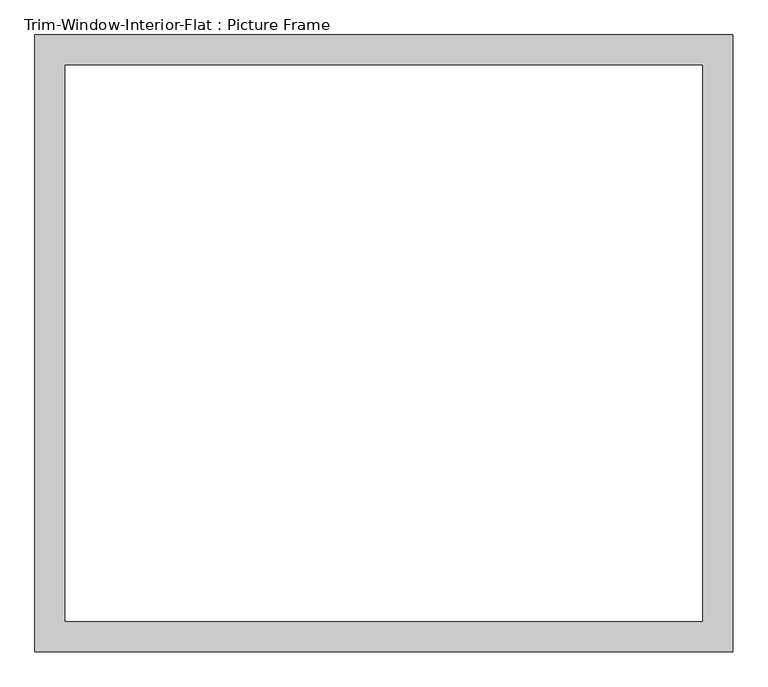
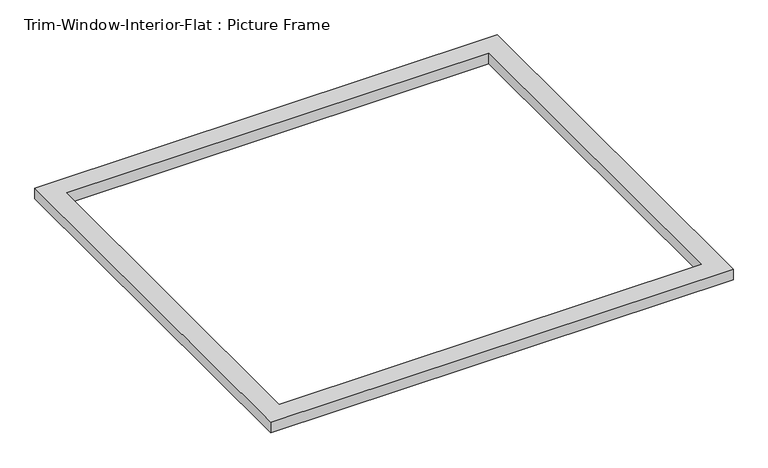
"""IFC4 building model written with IfcOpenShell, lengths in millimetres: proxy geometry, Trim-Window-Interior-Flat : Picture Frame."""

import ifcopenshell
import ifcopenshell.guid

model = None  # the IFC model being written
_history = None  # IfcOwnerHistory: only IFC2X3 demands one
_inside = {}  # id of a spatial element -> (the spatial element, [elements in it])
_under = {}  # id of a project, library or spatial element -> (it, [spatial elements below it])
_declared = {}  # id of a project -> (the project, [libraries it declares])
_typed = {}  # id of a type object -> (the type object, [elements of that type])
_made_of = {}  # id of a material, layer set ... -> (it, [elements and type objects made of it])


def new_model(schema):
    """Start an empty IFC model of exactly this schema.

    Asked for "IFC4X3", IfcOpenShell would pick the latest addendum, in which some entities
    have other attributes; the version numbers below select the first issue.
    IFC2X3 requires an IfcOwnerHistory on every rooted entity: one is made here for all.
    """
    global model, _history
    if schema == "IFC4X3":
        model = ifcopenshell.file(schema_version=(4, 3, 0, 0))
    else:
        model = ifcopenshell.file(schema=schema)
    _inside.clear()
    _under.clear()
    _declared.clear()
    _typed.clear()
    _made_of.clear()
    _history = None
    if model.schema == "IFC2X3":
        org = make("IfcOrganization", Name="unknown")
        user = make(
            "IfcPersonAndOrganization",
            ThePerson=make("IfcPerson", FamilyName="unknown"),
            TheOrganization=org,
        )
        app = make(
            "IfcApplication",
            ApplicationDeveloper=org,
            Version="unknown",
            ApplicationFullName="unknown",
            ApplicationIdentifier="unknown",
        )
        _history = make(
            "IfcOwnerHistory",
            OwningUser=user,
            OwningApplication=app,
            ChangeAction="ADDED",
            CreationDate=0,
        )
    return model


def make(cls, **values):
    """One entity of the class cls with the attributes given. An attribute that is None is left unset."""
    return model.create_entity(
        cls, **{name: value for name, value in values.items() if value is not None}
    )


def rooted(cls, **values):
    """An entity with a GlobalId (a new one), such as an element, a storey or a relation."""
    return make(cls, GlobalId=ifcopenshell.guid.new(), OwnerHistory=_history, **values)


def si_unit(unit_type, name, prefix=None):
    """IfcSIUnit, for example si_unit("LENGTHUNIT", "METRE", prefix="MILLI")."""
    return make("IfcSIUnit", UnitType=unit_type, Prefix=prefix, Name=name)


def assignment(units):
    """IfcUnitAssignment: the units of a project."""
    return None if units is None else make("IfcUnitAssignment", Units=units)


def point(xyz):
    """IfcCartesianPoint."""
    return None if xyz is None else make("IfcCartesianPoint", Coordinates=xyz)


def direction(xyz):
    """IfcDirection."""
    return None if xyz is None else make("IfcDirection", DirectionRatios=xyz)


def frame(location, z_axis=None, x_axis=None):
    """IfcAxis2Placement3D, a coordinate frame: its origin and axes. An axis left out is left unset."""
    return make(
        "IfcAxis2Placement3D",
        Location=point(location),
        Axis=direction(z_axis),
        RefDirection=direction(x_axis),
    )


def origin():
    """The frame at (0, 0, 0) with its axes left unset."""
    return frame((0.0, 0.0, 0.0))


def origin_with_axes():
    """The frame at (0, 0, 0) with the z axis (0, 0, 1) and the x axis (1, 0, 0) written out."""
    return frame((0.0, 0.0, 0.0), z_axis=(0.0, 0.0, 1.0), x_axis=(1.0, 0.0, 0.0))


def place(relative_to, where):
    """IfcLocalPlacement: puts the frame where relative to a parent placement (None: the world)."""
    return make(
        "IfcLocalPlacement", PlacementRelTo=relative_to, RelativePlacement=where
    )


def context(
    kind, dimensions, precision=None, world=None, true_north=None, identifier=None
):
    """IfcGeometricRepresentationContext, for example the 3D "Model" context."""
    return make(
        "IfcGeometricRepresentationContext",
        ContextIdentifier=identifier,
        ContextType=kind,
        CoordinateSpaceDimension=dimensions,
        Precision=precision,
        WorldCoordinateSystem=world,
        TrueNorth=true_north,
    )


def project(units=None, contexts=None):
    """IfcProject with its units and contexts."""
    return rooted(
        "IfcProject",
        Name="project",
        RepresentationContexts=contexts,
        UnitsInContext=assignment(units),
    )


def spatial(cls, under=None, at=None, **own):
    """A site, building, storey or space (cls), placed at a placement, below another one or the project."""
    s = rooted(cls, ObjectPlacement=at, **own)
    if under is not None:
        _under.setdefault(under.id(), (under, []))[1].append(s)
    return s


def polyline(points):
    """IfcPolyline through the points."""
    return make("IfcPolyline", Points=[point(p) for p in points])


def outline(outer, holes=None, kind="AREA"):
    """IfcArbitraryClosedProfileDef: a profile drawn as a closed curve; with holes, ...WithVoids."""
    if holes is None:
        return make("IfcArbitraryClosedProfileDef", ProfileType=kind, OuterCurve=outer)
    return make(
        "IfcArbitraryProfileDefWithVoids",
        ProfileType=kind,
        OuterCurve=outer,
        InnerCurves=holes,
    )


def extrude(swept, where, along, depth):
    """IfcExtrudedAreaSolid: the profile swept, set in the frame where, extruded along a direction by depth."""
    return make(
        "IfcExtrudedAreaSolid",
        SweptArea=swept,
        Position=where,
        ExtrudedDirection=direction(along),
        Depth=depth,
    )


def shape(context_of_items, identifier, shape_type, items):
    """IfcShapeRepresentation: the items that make up one representation, for example the "Body"."""
    return make(
        "IfcShapeRepresentation",
        ContextOfItems=context_of_items,
        RepresentationIdentifier=identifier,
        RepresentationType=shape_type,
        Items=items,
    )


def source(mapping_origin, context_of_items, identifier, shape_type, items):
    """IfcRepresentationMap: a shape defined once, which mapped items show again and again."""
    return make(
        "IfcRepresentationMap",
        MappingOrigin=mapping_origin,
        MappedRepresentation=shape(context_of_items, identifier, shape_type, items),
    )


def transform(
    local_origin,
    x_axis=None,
    y_axis=None,
    z_axis=None,
    scale=None,
    scale2=None,
    scale3=None,
    uniform=True,
):
    """IfcCartesianTransformationOperator3D, or its non-uniform kind. x_axis, y_axis, z_axis: its Axis1, 2, 3."""
    if uniform:
        return make(
            "IfcCartesianTransformationOperator3D",
            Axis1=direction(x_axis),
            Axis2=direction(y_axis),
            LocalOrigin=point(local_origin),
            Scale=scale,
            Axis3=direction(z_axis),
        )
    return make(
        "IfcCartesianTransformationOperator3DnonUniform",
        Axis1=direction(x_axis),
        Axis2=direction(y_axis),
        LocalOrigin=point(local_origin),
        Scale=scale,
        Axis3=direction(z_axis),
        Scale2=scale2,
        Scale3=scale3,
    )


def mapped(mapping_source, mapping_target):
    """IfcMappedItem: shows the shape of a source again, moved by a transform."""
    return make(
        "IfcMappedItem", MappingSource=mapping_source, MappingTarget=mapping_target
    )


def made_of(thing, what):
    """Note that an element or type object is made of a material, layer set ...; save() writes the relation."""
    if what is not None:
        _made_of.setdefault(what.id(), (what, []))[1].append(thing)
    return thing


def element(
    cls,
    number,
    at=None,
    inside=None,
    cuts=None,
    type_object=None,
    material=None,
    context=None,
    identifier="Body",
    shape_type=None,
    held_by="IfcProductDefinitionShape",
    body=None,
    shapes=None,
    **own,
):
    """One element of the class cls, such as IfcWall. Its Tag is "e" and its number.

    at: its placement. inside: the storey or other place that contains it. cuts: it is an
    opening in that element (IfcRelVoidsElement). A single representation is given by context,
    identifier, shape_type and body (its items); several are given by shapes. held_by: the class
    of the entity that holds the representations. save() writes the other relations.
    """
    e = rooted(cls, Tag="e%d" % number, ObjectPlacement=at, **own)
    if body is not None:
        shapes = [shape(context, identifier, shape_type, body)]
    if shapes is not None:
        e.Representation = make(held_by, Representations=shapes)
    if inside is not None:
        _inside.setdefault(inside.id(), (inside, []))[1].append(e)
    if cuts is not None:
        rooted(
            "IfcRelVoidsElement", RelatingBuildingElement=cuts, RelatedOpeningElement=e
        )
    if type_object is not None:
        _typed.setdefault(type_object.id(), (type_object, []))[1].append(e)
    return made_of(e, material)


def aggregate(whole, parts):
    """IfcRelAggregates: a whole, such as a stair, and the parts it consists of."""
    return rooted("IfcRelAggregates", RelatingObject=whole, RelatedObjects=parts)


def save(model, path):
    """Write the relations noted so far, then the file.

    IfcRelAggregates (storeys below a building ...), IfcRelContainedInSpatialStructure (elements
    in a storey), IfcRelDefinesByType, IfcRelAssociatesMaterial and IfcRelDeclares: one each for
    every whole, place, type object, material and project.
    """
    for whole, parts in _under.values():
        aggregate(whole, parts)
    for where, things in _inside.values():
        rooted(
            "IfcRelContainedInSpatialStructure",
            RelatedElements=things,
            RelatingStructure=where,
        )
    for kind, things in _typed.values():
        rooted("IfcRelDefinesByType", RelatedObjects=things, RelatingType=kind)
    for what, things in _made_of.values():
        rooted("IfcRelAssociatesMaterial", RelatedObjects=things, RelatingMaterial=what)
    for by, libraries in _declared.values():
        rooted("IfcRelDeclares", RelatingContext=by, RelatedDefinitions=libraries)
    model.write(path)


def trim_window_interior_flat_picture_frame_1dce1945(model_context):
    return source(origin(), model_context, "Body", "SweptSolid", [
        extrude(outline(polyline([(654.05, 44.45), (654.05, -1111.25), (-654.05, -1111.25), (-654.05, 44.45), (654.05, 44.45)]), holes=[polyline([(596.9, -12.7), (-596.9, -12.7), (-596.9, -1054.1), (596.9, -1054.1), (596.9, -12.7)])]), origin_with_axes(), (0.0, 0.0, 1.0), 31.75),
    ])


if __name__ == "__main__":
    model = new_model("IFC4")
    model_context = context("Model", 3, world=origin())
    ifc_project = project(units=[si_unit("LENGTHUNIT", "METRE", prefix="MILLI")], contexts=[model_context])
    site = spatial("IfcSite", under=ifc_project)
    building = spatial("IfcBuilding", under=site)
    placement = place(None, origin())
    trim_window_interior_flat_picture_frame_shape = trim_window_interior_flat_picture_frame_1dce1945(model_context)
    element("IfcBuildingElementProxy", 1, Name="Trim-Window-Interior-Flat : Picture Frame", ObjectType="Trim-Window-Interior-Flat : Picture Frame", at=placement, inside=building, context=model_context, shape_type="MappedRepresentation", body=[
        mapped(trim_window_interior_flat_picture_frame_shape, transform((0.0, 0.0, 0.0), x_axis=(1.0, 0.0, 0.0), y_axis=(0.0, 1.0, 0.0), z_axis=(0.0, 0.0, 1.0))),
    ])
    save(model, "model.ifc")

# Revit data of these elements
# Type "Trim-Window-Interior-Flat : Picture Frame"
#   Trim Thickness_Picture Frame = 3.175 cm
#   Trim Width = 5.715 cm
#   Trim Thickness_with Sill = 1.905 cm
#   Sill Thickness = 3.175 cm
#   Opening Width [instance default] = 60.96 cm
#   Opening Height [instance default] = 91.44 cm
#   Default Elevation = 121.92 cm
#   Sill = no
#   Picture Frame = yes
#   Trim Material [instance default] = none
# Element 1 (IfcBuildingElementProxy, "Trim-Window-Interior-Flat : Picture Frame")
#   Opening Width = 121.92 cm
#   Opening Height = 106.68 cm
#   Trim Material = Wood - Stained
#   Materials on its faces: "Wood - Stained"
# Materials
#   "Wood - Stained": class "Wood", colour RGB 224 178 126, transparency 0, Cost = 0
